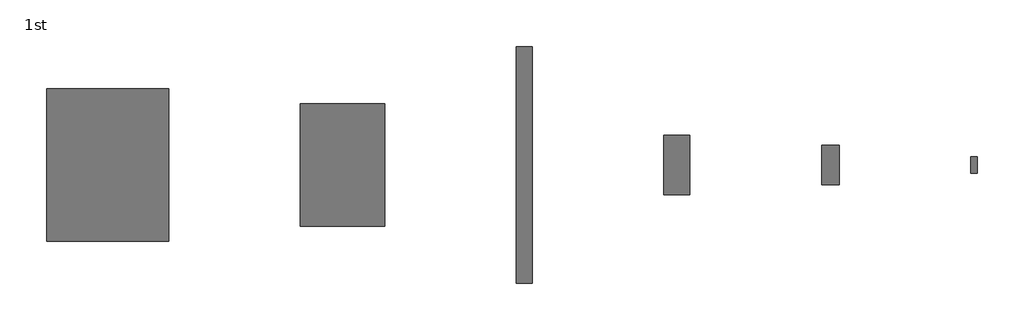
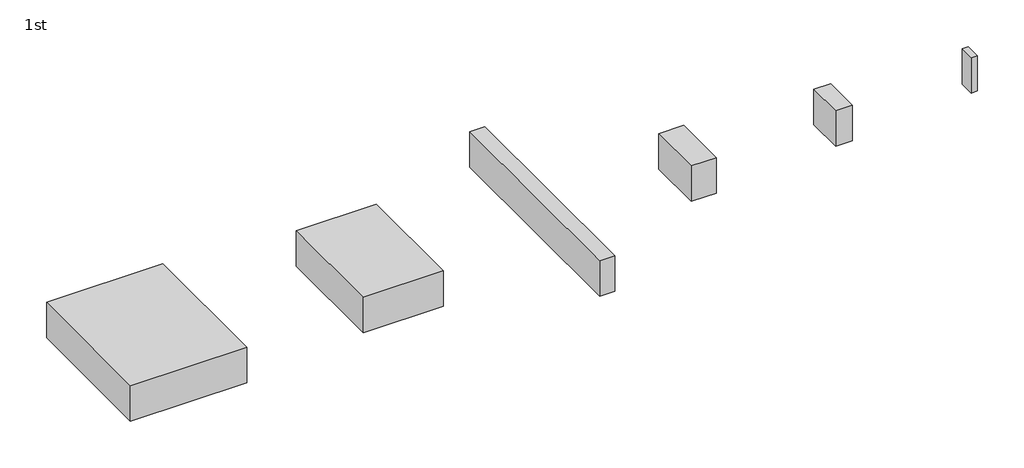
# One storey: 6 proxies.
"""IFC4 building model written with IfcOpenShell, lengths in millimetres."""

import ifcopenshell
import ifcopenshell.guid

model = None  # the IFC model being written
_history = None  # IfcOwnerHistory: only IFC2X3 demands one
_inside = {}  # id of a spatial element -> (the spatial element, [elements in it])
_under = {}  # id of a project, library or spatial element -> (it, [spatial elements below it])
_declared = {}  # id of a project -> (the project, [libraries it declares])
_typed = {}  # id of a type object -> (the type object, [elements of that type])
_made_of = {}  # id of a material, layer set ... -> (it, [elements and type objects made of it])


def new_model(schema):
    """Start an empty IFC model of exactly this schema.

    Asked for "IFC4X3", IfcOpenShell would pick the latest addendum, in which some entities
    have other attributes; the version numbers below select the first issue.
    IFC2X3 requires an IfcOwnerHistory on every rooted entity: one is made here for all.
    """
    global model, _history
    if schema == "IFC4X3":
        model = ifcopenshell.file(schema_version=(4, 3, 0, 0))
    else:
        model = ifcopenshell.file(schema=schema)
    _inside.clear()
    _under.clear()
    _declared.clear()
    _typed.clear()
    _made_of.clear()
    _history = None
    if model.schema == "IFC2X3":
        org = make("IfcOrganization", Name="unknown")
        user = make(
            "IfcPersonAndOrganization",
            ThePerson=make("IfcPerson", FamilyName="unknown"),
            TheOrganization=org,
        )
        app = make(
            "IfcApplication",
            ApplicationDeveloper=org,
            Version="unknown",
            ApplicationFullName="unknown",
            ApplicationIdentifier="unknown",
        )
        _history = make(
            "IfcOwnerHistory",
            OwningUser=user,
            OwningApplication=app,
            ChangeAction="ADDED",
            CreationDate=0,
        )
    return model


def make(cls, **values):
    """One entity of the class cls with the attributes given. An attribute that is None is left unset."""
    return model.create_entity(
        cls, **{name: value for name, value in values.items() if value is not None}
    )


def rooted(cls, **values):
    """An entity with a GlobalId (a new one), such as an element, a storey or a relation."""
    return make(cls, GlobalId=ifcopenshell.guid.new(), OwnerHistory=_history, **values)


def si_unit(unit_type, name, prefix=None):
    """IfcSIUnit, for example si_unit("LENGTHUNIT", "METRE", prefix="MILLI")."""
    return make("IfcSIUnit", UnitType=unit_type, Prefix=prefix, Name=name)


def assignment(units):
    """IfcUnitAssignment: the units of a project."""
    return None if units is None else make("IfcUnitAssignment", Units=units)


def point(xyz):
    """IfcCartesianPoint."""
    return None if xyz is None else make("IfcCartesianPoint", Coordinates=xyz)


def direction(xyz):
    """IfcDirection."""
    return None if xyz is None else make("IfcDirection", DirectionRatios=xyz)


def frame(location, z_axis=None, x_axis=None):
    """IfcAxis2Placement3D, a coordinate frame: its origin and axes. An axis left out is left unset."""
    return make(
        "IfcAxis2Placement3D",
        Location=point(location),
        Axis=direction(z_axis),
        RefDirection=direction(x_axis),
    )


def origin():
    """The frame at (0, 0, 0) with its axes left unset."""
    return frame((0.0, 0.0, 0.0))


def origin_with_axes():
    """The frame at (0, 0, 0) with the z axis (0, 0, 1) and the x axis (1, 0, 0) written out."""
    return frame((0.0, 0.0, 0.0), z_axis=(0.0, 0.0, 1.0), x_axis=(1.0, 0.0, 0.0))


def place(relative_to, where):
    """IfcLocalPlacement: puts the frame where relative to a parent placement (None: the world)."""
    return make(
        "IfcLocalPlacement", PlacementRelTo=relative_to, RelativePlacement=where
    )


def context(
    kind, dimensions, precision=None, world=None, true_north=None, identifier=None
):
    """IfcGeometricRepresentationContext, for example the 3D "Model" context."""
    return make(
        "IfcGeometricRepresentationContext",
        ContextIdentifier=identifier,
        ContextType=kind,
        CoordinateSpaceDimension=dimensions,
        Precision=precision,
        WorldCoordinateSystem=world,
        TrueNorth=true_north,
    )


def project(units=None, contexts=None):
    """IfcProject with its units and contexts."""
    return rooted(
        "IfcProject",
        Name="project",
        RepresentationContexts=contexts,
        UnitsInContext=assignment(units),
    )


def spatial(cls, under=None, at=None, **own):
    """A site, building, storey or space (cls), placed at a placement, below another one or the project."""
    s = rooted(cls, ObjectPlacement=at, **own)
    if under is not None:
        _under.setdefault(under.id(), (under, []))[1].append(s)
    return s


def polyline(points):
    """IfcPolyline through the points."""
    return make("IfcPolyline", Points=[point(p) for p in points])


def outline(outer, holes=None, kind="AREA"):
    """IfcArbitraryClosedProfileDef: a profile drawn as a closed curve; with holes, ...WithVoids."""
    if holes is None:
        return make("IfcArbitraryClosedProfileDef", ProfileType=kind, OuterCurve=outer)
    return make(
        "IfcArbitraryProfileDefWithVoids",
        ProfileType=kind,
        OuterCurve=outer,
        InnerCurves=holes,
    )


def extrude(swept, where, along, depth):
    """IfcExtrudedAreaSolid: the profile swept, set in the frame where, extruded along a direction by depth."""
    return make(
        "IfcExtrudedAreaSolid",
        SweptArea=swept,
        Position=where,
        ExtrudedDirection=direction(along),
        Depth=depth,
    )


def shape(context_of_items, identifier, shape_type, items):
    """IfcShapeRepresentation: the items that make up one representation, for example the "Body"."""
    return make(
        "IfcShapeRepresentation",
        ContextOfItems=context_of_items,
        RepresentationIdentifier=identifier,
        RepresentationType=shape_type,
        Items=items,
    )


def source(mapping_origin, context_of_items, identifier, shape_type, items):
    """IfcRepresentationMap: a shape defined once, which mapped items show again and again."""
    return make(
        "IfcRepresentationMap",
        MappingOrigin=mapping_origin,
        MappedRepresentation=shape(context_of_items, identifier, shape_type, items),
    )


def transform(
    local_origin,
    x_axis=None,
    y_axis=None,
    z_axis=None,
    scale=None,
    scale2=None,
    scale3=None,
    uniform=True,
):
    """IfcCartesianTransformationOperator3D, or its non-uniform kind. x_axis, y_axis, z_axis: its Axis1, 2, 3."""
    if uniform:
        return make(
            "IfcCartesianTransformationOperator3D",
            Axis1=direction(x_axis),
            Axis2=direction(y_axis),
            LocalOrigin=point(local_origin),
            Scale=scale,
            Axis3=direction(z_axis),
        )
    return make(
        "IfcCartesianTransformationOperator3DnonUniform",
        Axis1=direction(x_axis),
        Axis2=direction(y_axis),
        LocalOrigin=point(local_origin),
        Scale=scale,
        Axis3=direction(z_axis),
        Scale2=scale2,
        Scale3=scale3,
    )


def mapped(mapping_source, mapping_target):
    """IfcMappedItem: shows the shape of a source again, moved by a transform."""
    return make(
        "IfcMappedItem", MappingSource=mapping_source, MappingTarget=mapping_target
    )


def made_of(thing, what):
    """Note that an element or type object is made of a material, layer set ...; save() writes the relation."""
    if what is not None:
        _made_of.setdefault(what.id(), (what, []))[1].append(thing)
    return thing


def element(
    cls,
    number,
    at=None,
    inside=None,
    cuts=None,
    type_object=None,
    material=None,
    context=None,
    identifier="Body",
    shape_type=None,
    held_by="IfcProductDefinitionShape",
    body=None,
    shapes=None,
    **own,
):
    """One element of the class cls, such as IfcWall. Its Tag is "e" and its number.

    at: its placement. inside: the storey or other place that contains it. cuts: it is an
    opening in that element (IfcRelVoidsElement). A single representation is given by context,
    identifier, shape_type and body (its items); several are given by shapes. held_by: the class
    of the entity that holds the representations. save() writes the other relations.
    """
    e = rooted(cls, Tag="e%d" % number, ObjectPlacement=at, **own)
    if body is not None:
        shapes = [shape(context, identifier, shape_type, body)]
    if shapes is not None:
        e.Representation = make(held_by, Representations=shapes)
    if inside is not None:
        _inside.setdefault(inside.id(), (inside, []))[1].append(e)
    if cuts is not None:
        rooted(
            "IfcRelVoidsElement", RelatingBuildingElement=cuts, RelatedOpeningElement=e
        )
    if type_object is not None:
        _typed.setdefault(type_object.id(), (type_object, []))[1].append(e)
    return made_of(e, material)


def aggregate(whole, parts):
    """IfcRelAggregates: a whole, such as a stair, and the parts it consists of."""
    return rooted("IfcRelAggregates", RelatingObject=whole, RelatedObjects=parts)


def save(model, path):
    """Write the relations noted so far, then the file.

    IfcRelAggregates (storeys below a building ...), IfcRelContainedInSpatialStructure (elements
    in a storey), IfcRelDefinesByType, IfcRelAssociatesMaterial and IfcRelDeclares: one each for
    every whole, place, type object, material and project.
    """
    for whole, parts in _under.values():
        aggregate(whole, parts)
    for where, things in _inside.values():
        rooted(
            "IfcRelContainedInSpatialStructure",
            RelatedElements=things,
            RelatingStructure=where,
        )
    for kind, things in _typed.values():
        rooted("IfcRelDefinesByType", RelatedObjects=things, RelatingType=kind)
    for what, things in _made_of.values():
        rooted("IfcRelAssociatesMaterial", RelatedObjects=things, RelatingMaterial=what)
    for by, libraries in _declared.values():
        rooted("IfcRelDeclares", RelatingContext=by, RelatedDefinitions=libraries)
    model.write(path)


def space_planning_box_space_planning_box_29bcd6f9(model_context):
    return source(origin(), model_context, "Body", "SweptSolid", [
        extrude(outline(polyline([(2000.0, 4500.0), (2000.0, -4500.0), (-2000.0, -4500.0), (-2000.0, 4500.0), (2000.0, 4500.0)])), origin_with_axes(), (0.0, 0.0, 1.0), 6000.0),
    ])


def space_planning_box_space_planning_box_d82b1902(model_context):
    return source(origin(), model_context, "Body", "SweptSolid", [
        extrude(outline(polyline([(9300.0, 11600.0), (9300.0, -11600.0), (-9300.0, -11600.0), (-9300.0, 11600.0), (9300.0, 11600.0)])), origin_with_axes(), (0.0, 0.0, 1.0), 6000.0),
    ])


def space_planning_box_space_planning_box_21711933(model_context):
    return source(origin(), model_context, "Body", "SweptSolid", [
        extrude(outline(polyline([(6400.0, 9300.0), (6400.0, -9300.0), (-6400.0, -9300.0), (-6400.0, 9300.0), (6400.0, 9300.0)])), origin_with_axes(), (0.0, 0.0, 1.0), 6000.0),
    ])


def space_planning_box_space_planning_box_03d31222(model_context):
    return source(origin(), model_context, "Body", "SweptSolid", [
        extrude(outline(polyline([(1200.0, 18000.0), (1200.0, -18000.0), (-1200.0, -18000.0), (-1200.0, 18000.0), (1200.0, 18000.0)])), origin_with_axes(), (0.0, 0.0, 1.0), 6000.0),
    ])


def space_planning_box_space_planning_box_5634f436(model_context):
    return source(origin(), model_context, "Body", "SweptSolid", [
        extrude(outline(polyline([(1350.0, 3000.0), (1350.0, -3000.0), (-1350.0, -3000.0), (-1350.0, 3000.0), (1350.0, 3000.0)])), origin_with_axes(), (0.0, 0.0, 1.0), 6000.0),
    ])


def space_planning_box_space_planning_box_71e2440f(model_context):
    return source(origin(), model_context, "Body", "SweptSolid", [
        extrude(outline(polyline([(500.0, 1250.0), (500.0, -1250.0), (-500.0, -1250.0), (-500.0, 1250.0), (500.0, 1250.0)])), origin_with_axes(), (0.0, 0.0, 1.0), 6000.0),
    ])


model = new_model("IFC4")

# Units and contexts
model_context = context("Model", 3, world=origin())
ifc_project = project(units=[si_unit("LENGTHUNIT", "METRE", prefix="MILLI")], contexts=[model_context])

# Site, building, storey
site = spatial("IfcSite", under=ifc_project)
building = spatial("IfcBuilding", under=site)
storey = spatial("IfcBuildingStorey", under=building, Name="1st", Elevation=7000.0)

# Proxies
placement = place(None, origin())
space_planning_box_space_planning_box_shape = space_planning_box_space_planning_box_29bcd6f9(model_context)
element("IfcBuildingElementProxy", 1, Name="Space Planning Box : Space Planning Box", ObjectType="Space Planning Box : Space Planning Box", at=placement, inside=storey, context=model_context, shape_type="MappedRepresentation", body=[
    mapped(space_planning_box_space_planning_box_shape, transform((95800.0, 114000.0, 7000.0), x_axis=(1.0, 0.0, 0.0), y_axis=(0.0, 1.0, 0.0), z_axis=(0.0, 0.0, 1.0))),
])
space_planning_box_space_planning_box_2_shape = space_planning_box_space_planning_box_d82b1902(model_context)
element("IfcBuildingElementProxy", 2, Name="Space Planning Box : Space Planning Box", ObjectType="Space Planning Box : Space Planning Box", at=placement, inside=storey, context=model_context, shape_type="MappedRepresentation", body=[
    mapped(space_planning_box_space_planning_box_2_shape, transform((9300.0, 114000.0, 7000.0), x_axis=(1.0, 0.0, 0.0), y_axis=(0.0, 1.0, 0.0), z_axis=(0.0, 0.0, 1.0))),
])
space_planning_box_space_planning_box_3_shape = space_planning_box_space_planning_box_21711933(model_context)
element("IfcBuildingElementProxy", 3, Name="Space Planning Box : Space Planning Box", ObjectType="Space Planning Box : Space Planning Box", at=placement, inside=storey, context=model_context, shape_type="MappedRepresentation", body=[
    mapped(space_planning_box_space_planning_box_3_shape, transform((45000.0, 114000.0, 7000.0), x_axis=(1.0, 0.0, 0.0), y_axis=(0.0, 1.0, 0.0), z_axis=(0.0, 0.0, 1.0))),
])
space_planning_box_space_planning_box_4_shape = space_planning_box_space_planning_box_03d31222(model_context)
element("IfcBuildingElementProxy", 4, Name="Space Planning Box : Space Planning Box", ObjectType="Space Planning Box : Space Planning Box", at=placement, inside=storey, context=model_context, shape_type="MappedRepresentation", body=[
    mapped(space_planning_box_space_planning_box_4_shape, transform((72600.0, 114000.0, 7000.0), x_axis=(1.0, 0.0, 0.0), y_axis=(0.0, 1.0, 0.0), z_axis=(0.0, 0.0, 1.0))),
])
space_planning_box_space_planning_box_5_shape = space_planning_box_space_planning_box_5634f436(model_context)
element("IfcBuildingElementProxy", 5, Name="Space Planning Box : Space Planning Box", ObjectType="Space Planning Box : Space Planning Box", at=placement, inside=storey, context=model_context, shape_type="MappedRepresentation", body=[
    mapped(space_planning_box_space_planning_box_5_shape, transform((119150.0, 114000.0, 7000.0), x_axis=(1.0, 0.0, 0.0), y_axis=(0.0, 1.0, 0.0), z_axis=(0.0, 0.0, 1.0))),
])
space_planning_box_space_planning_box_6_shape = space_planning_box_space_planning_box_71e2440f(model_context)
element("IfcBuildingElementProxy", 6, Name="Space Planning Box : Space Planning Box", ObjectType="Space Planning Box : Space Planning Box", at=placement, inside=storey, context=model_context, shape_type="MappedRepresentation", body=[
    mapped(space_planning_box_space_planning_box_6_shape, transform((141000.0, 114000.0, 7000.0), x_axis=(1.0, 0.0, 0.0), y_axis=(0.0, 1.0, 0.0), z_axis=(0.0, 0.0, 1.0))),
])

save(model, "model.ifc")

# Revit data of these elements
# Project information
#   Project Issue Date = "Issue Date"
#   Project Status = "Project Status"
#   Client Name = "Owner"
#   Project Address = "Enter address here"
#   Project Name = "Project Name"
#   Project Number = "Project Number"
# Type "Space Planning Box : Space Planning Box"
#   Type Comments = "..."
#   Room Name [instance default] = "?"
#   Assembly Code = "..."
#   Width [instance default] = 1524 mm
#   Program Area [instance default] = 0 m²
#   Length [instance default] = 1524 mm
#   Height [instance default] = 1524 mm
#   Area [instance default] = 2.32258 m²
#   Fill Color [instance default] = Cyan
#   Default Elevation = 0
# Element 1 (IfcBuildingElementProxy, "Space Planning Box : Space Planning Box")
#   Room Name = "Stairway"
#   Width = 4000 mm
#   Program Area = 36 m²
#   Length = 9000 mm
#   Height = 6000 mm
#   Area = 36 m²
#   Fill Color = Lavender
#   Phase Created = New Construction
#   Materials on its faces: "Lavender"
# Element 2 (IfcBuildingElementProxy, "Space Planning Box : Space Planning Box")
#   Room Name = "Electronic Room"
#   Width = 18600 mm
#   Program Area = 431.52 m²
#   Length = 23200 mm
#   Height = 6000 mm
#   Area = 431.52 m²
#   Fill Color = Lime
#   Phase Created = New Construction
#   Materials on its faces: "Lime"
# Element 3 (IfcBuildingElementProxy, "Space Planning Box : Space Planning Box")
#   Room Name = "Electrical Room"
#   Width = 12800 mm
#   Program Area = 238.08 m²
#   Length = 18600 mm
#   Height = 6000 mm
#   Area = 238.08 m²
#   Fill Color = Blue
#   Phase Created = New Construction
#   Materials on its faces: "Blue"
# Element 4 (IfcBuildingElementProxy, "Space Planning Box : Space Planning Box")
#   Room Name = "Corridor"
#   Width = 2400 mm
#   Program Area = 86.4 m²
#   Length = 36000 mm
#   Height = 6000 mm
#   Area = 86.4 m²
#   Fill Color = Lavender
#   Phase Created = New Construction
#   Materials on its faces: "Lavender"
# Element 5 (IfcBuildingElementProxy, "Space Planning Box : Space Planning Box")
#   Room Name = "Duct Shaft"
#   Width = 2700 mm
#   Program Area = 16.2 m²
#   Length = 6000 mm
#   Height = 6000 mm
#   Area = 16.2 m²
#   Fill Color = Pink
#   Phase Created = New Construction
#   Materials on its faces: "Pink"
# Element 6 (IfcBuildingElementProxy, "Space Planning Box : Space Planning Box")
#   Room Name = "Pipe Shaft"
#   Width = 1000 mm
#   Program Area = 2.5 m²
#   Length = 2500 mm
#   Height = 6000 mm
#   Area = 2.5 m²
#   Fill Color = Pink
#   Phase Created = New Construction
#   Materials on its faces: "Pink"
# Materials
#   "Cyan": class "Generic", colour RGB 0 255 255, transparency 0.2, Cost = 0
#   "Lavender": class "Generic", colour RGB 186 85 211, transparency 0.2, Cost = 0
#   "Lime": class "Generic", colour RGB 0 255 0, transparency 0.2, Cost = 0
#   "Blue": class "Generic", colour RGB 0 0 255, transparency 0.2, Cost = 0
#   "Pink": class "Generic", colour RGB 255 105 180, transparency 0.2, Cost = 0
